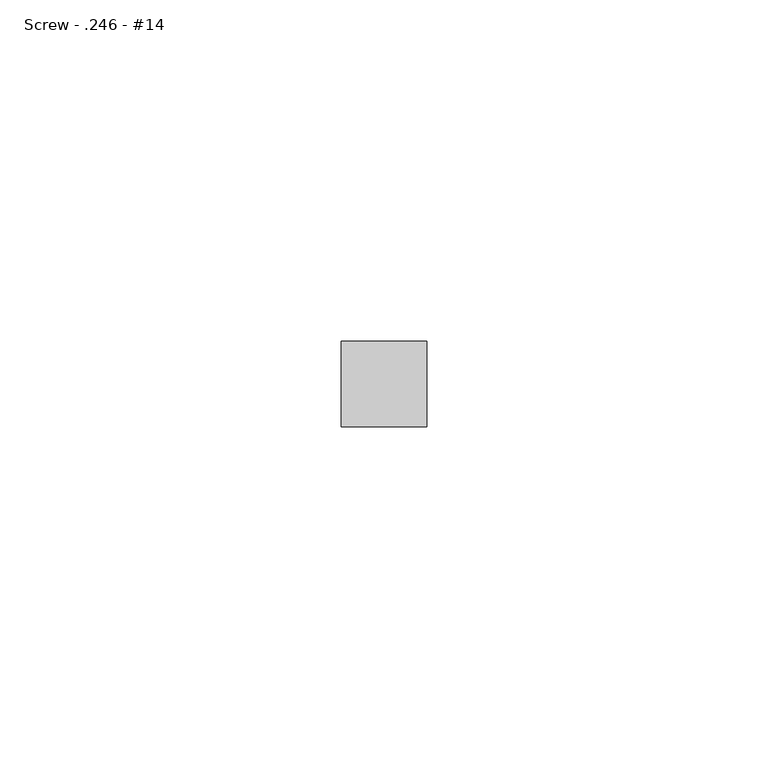
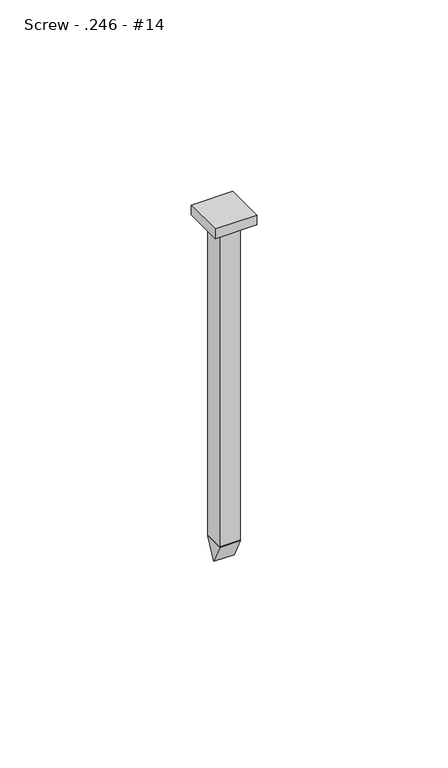
"""IFC4 building model written with IfcOpenShell, lengths in millimetres: fastener geometry, 060523 - W_P_C - Fastenings - Generic - SQUARE : Screw - .246 - #14."""

from ifc_helpers import new_model, si_unit, frame, origin, origin_with_axes, place, context, project, spatial, polyline, outline, extrude, source, transform, mapped, element, save


def screw_246_14_be59b448(model_context):
    return source(origin(), model_context, "Body", "SweptSolid", [
        extrude(outline(polyline([(0.0, -107.8484), (-3.1242, -101.6), (3.1242, -101.6), (0.0, -107.8484)])), frame((-3.1242, 0.0, 0.0), z_axis=(1.0, 0.0, 0.0), x_axis=(0.0, 1.0, 0.0)), (0.0, 0.0, 1.0), 6.2484),
        extrude(outline(polyline([(-6.2484, -6.2484), (-6.2484, 6.2484), (6.2484, 6.2484), (6.2484, -6.2484), (-6.2484, -6.2484)])), origin_with_axes(), (0.0, 0.0, 1.0), 3.1242),
        extrude(outline(polyline([(-3.1242, 3.1242), (3.1242, 3.1242), (3.1242, -3.1242), (-3.1242, -3.1242), (-3.1242, 3.1242)])), frame((0.0, 0.0, -101.6), z_axis=(0.0, 0.0, 1.0), x_axis=(1.0, 0.0, 0.0)), (0.0, 0.0, 1.0), 101.6),
    ])


if __name__ == "__main__":
    model = new_model("IFC4")
    model_context = context("Model", 3, world=origin())
    ifc_project = project(units=[si_unit("LENGTHUNIT", "METRE", prefix="MILLI")], contexts=[model_context])
    site = spatial("IfcSite", under=ifc_project)
    building = spatial("IfcBuilding", under=site)
    placement = place(None, origin())
    screw_246_14_shape = screw_246_14_be59b448(model_context)
    element("IfcFastener", 1, ObjectType="060523 - W_P_C - Fastenings - Generic - SQUARE : Screw - .246 - #14", at=placement, inside=building, context=model_context, shape_type="MappedRepresentation", body=[
        mapped(screw_246_14_shape, transform((0.0, 0.0, 0.0), x_axis=(1.0, 0.0, 0.0), y_axis=(0.0, 1.0, 0.0), z_axis=(0.0, 0.0, 1.0))),
    ])
    save(model, "model.ifc")

# Revit data of these elements
# Type "060523 - W_P_C - Fastenings - Generic - SQUARE : Screw - .246 - #14"
#   Washer_Thickness = 0' - 0.00333"
#   Washer Radius = 0' - 0.133"
#   Washer Offset - Head = 0' - 0"
#   Washer Offset = 0' - 0"
#   Thickness_of_Substrate [instance default] = 0' - 1"
#   Side = 0' - 0 37/64"
#   Radius = 0' - 0.123"
#   Length [instance default] = 0' - 4"
#   Head Size = 0' - 1"
#   Head Radius = 0' - 0 1/2"
#   Head Height = 0' - 0.01"
#   Double Diameter = 0' - 0.492"
#   Diameter = 0' - 0.246"
#   Default Elevation = 4' - 0"
#   Washer_Nut_Visibility = no
#   Washer_Head_Visibility = no
#   Round_Head_Visibility = yes
#   Point Visibility = yes
#   Nut_Visibility = no
#   Hex_Head_Visiblilty = no
#   Washer Material = none
#   Bolt Material (Size) = AT SILL - FASTENER AT 24" O.C.
# Materials
#   "AT SILL - FASTENER AT 24\" O.C.": class "Generic", colour RGB 120 120 120, transparency 0, Cost = 0
